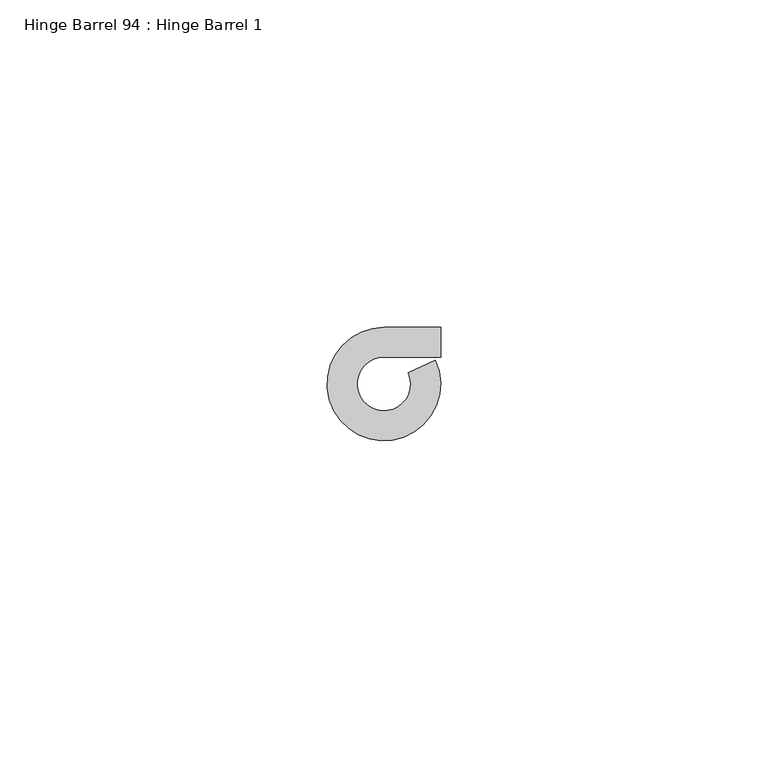
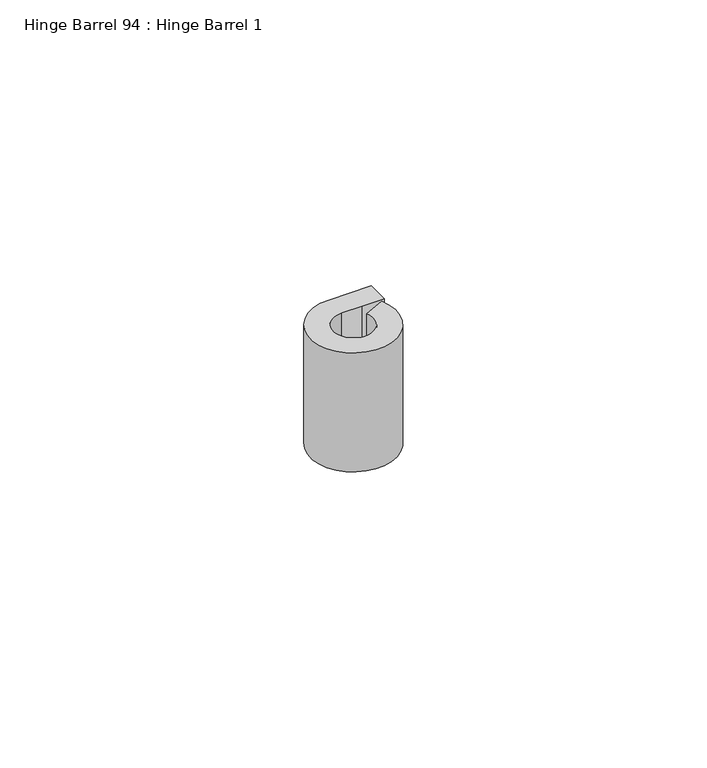
"""IFC4 building model written with IfcOpenShell, lengths in millimetres: proxy geometry, Hinge Barrel 94 : Hinge Barrel 1."""

from ifc_helpers import new_model, si_unit, point, frame, frame_2d, origin, place, context, project, spatial, polyline, circle_curve, trimmed, segment, composite_curve, outline, extrude, source, transform, mapped, element, save


def hinge_barrel_94_hinge_barrel_1_a937cab9(model_context):
    return source(origin(), model_context, "Body", "SweptSolid", [
        extrude(outline(composite_curve([segment(polyline([(587323.2214739, -533980.5883841), (587319.1320739, -533980.5883841)]), True, "CONTINUOUS"), segment(trimmed(circle_curve(frame_2d((587319.1320739, -533984.6777841)), 4.0894), [point((587319.1320739, -533980.5883841))], [point((587322.8436736, -533982.9610371))], True, "CARTESIAN"), True, "CONTINUOUS"), segment(polyline([(587322.8436736, -533982.9610371), (587326.986084, -533981.0450249)]), True, "CONTINUOUS"), segment(trimmed(circle_curve(frame_2d((587319.1320739, -533984.6777841)), 8.6534625), [point((587326.986084, -533981.0450249))], [point((587319.1320739, -533976.0243216))], False, "CARTESIAN"), True, "CONTINUOUS"), segment(polyline([(587319.1320739, -533976.0243216), (587327.7934739, -533976.0243216), (587327.7934739, -533980.5883841), (587323.2214739, -533980.5883841)]), True, "CONTINUOUS")], self_intersect=False)), frame((0.0, 0.0, 412.75), z_axis=(0.0, 0.0, 1.0), x_axis=(1.0, 0.0, 0.0)), (0.0, 0.0, 1.0), 25.4),
    ])


if __name__ == "__main__":
    model = new_model("IFC4")
    model_context = context("Model", 3, world=origin())
    ifc_project = project(units=[si_unit("LENGTHUNIT", "METRE", prefix="MILLI")], contexts=[model_context])
    site = spatial("IfcSite", under=ifc_project)
    building = spatial("IfcBuilding", under=site)
    placement = place(None, origin())
    hinge_barrel_94_hinge_barrel_1_shape = hinge_barrel_94_hinge_barrel_1_a937cab9(model_context)
    element("IfcBuildingElementProxy", 1, Name="Hinge Barrel 94 : Hinge Barrel 1", ObjectType="Hinge Barrel 94 : Hinge Barrel 1", at=placement, inside=building, context=model_context, shape_type="MappedRepresentation", body=[
        mapped(hinge_barrel_94_hinge_barrel_1_shape, transform((0.0, 0.0, 0.0), x_axis=(1.0, 0.0, 0.0), y_axis=(0.0, 1.0, 0.0), z_axis=(0.0, 0.0, 1.0))),
    ])
    save(model, "model.ifc")

# Revit data of these elements
# Element 1 (IfcBuildingElementProxy, "Hinge Barrel 94 : Hinge Barrel 1")
#   Materials on its faces: "6\"X6\" WELD-ON STL BUTT HINGE"
# Materials
#   "6\"X6\" WELD-ON STL BUTT HINGE": class "Metal", colour RGB 189 187 185, transparency 0, Description = "Carbon steel", Cost = 0
